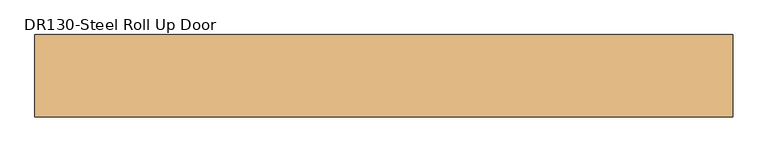
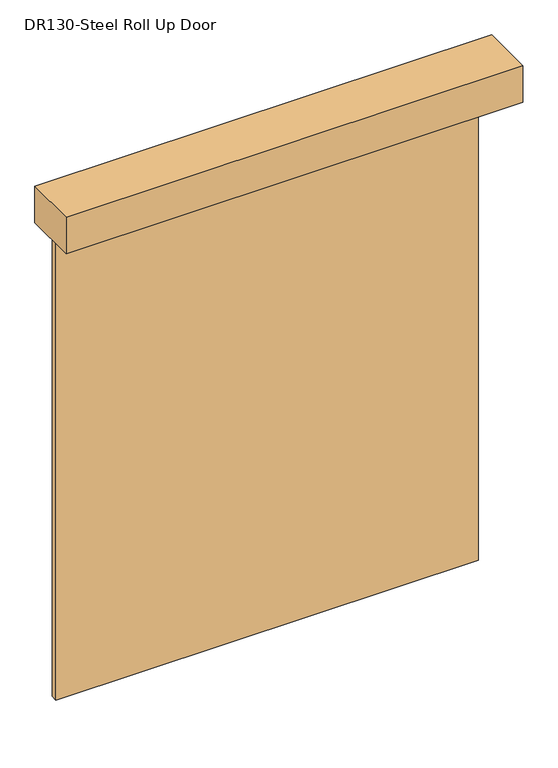
"""IFC4 building model written with IfcOpenShell, lengths in millimetres: door geometry, DR130-Steel Roll Up Door : DR131-Steel Roll Up Door-W4000xH4000mm."""

from ifc_helpers import new_model, si_unit, frame, origin, origin_with_axes, place, context, project, spatial, polyline, outline, extrude, source, transform, mapped, element, save


def dr130_steel_roll_up_door_e99b7ff9(model_context):
    return source(origin(), model_context, "Body", "SweptSolid", [
        extrude(outline(polyline([(2703.2, -858.8), (-2703.2, -858.8), (-2703.2, -220.0), (2703.2, -220.0), (2703.2, -858.8)])), frame((0.0, 0.0, 6000.0), z_axis=(0.0, 0.0, 1.0), x_axis=(1.0, 0.0, 0.0)), (0.0, 0.0, 1.0), 457.2),
        extrude(outline(polyline([(2500.0, -220.0), (2500.0, -300.0), (-2500.0, -300.0), (-2500.0, -220.0), (2500.0, -220.0)])), origin_with_axes(), (0.0, 0.0, 1.0), 6000.0),
    ])


if __name__ == "__main__":
    model = new_model("IFC4")
    model_context = context("Model", 3, world=origin())
    ifc_project = project(units=[si_unit("LENGTHUNIT", "METRE", prefix="MILLI")], contexts=[model_context])
    site = spatial("IfcSite", under=ifc_project)
    building = spatial("IfcBuilding", under=site)
    placement = place(None, origin())
    dr130_steel_roll_up_door_shape = dr130_steel_roll_up_door_e99b7ff9(model_context)
    element("IfcDoor", 1, ObjectType="DR130-Steel Roll Up Door : DR131-Steel Roll Up Door-W4000xH4000mm", at=placement, inside=building, context=model_context, shape_type="MappedRepresentation", body=[
        mapped(dr130_steel_roll_up_door_shape, transform((0.0, 0.0, 0.0), x_axis=(1.0, 0.0, 0.0), y_axis=(0.0, 1.0, 0.0), z_axis=(0.0, 0.0, 1.0))),
    ])
    save(model, "model.ifc")

# Revit data of these elements
# Type "DR130-Steel Roll Up Door : DR131-Steel Roll Up Door-W4000xH4000mm"
#   Type Mark = "362"
#   Construction Type Id = "MDOOR"
#   Assembly Code = "B2030400"
#   Analytic Construction = "<None>"
#   Thickness = 0.0800 m
#   Thermal Resistance (R) = 0.270117 (m²·K)/W
#   Rough Width [instance default] = 4.0000 m
#   Rough Height [instance default] = 4.0000 m
#   Offset [instance default] = 1.0000 m
#   Heat Transfer Coefficient (U) = 3.7021 W/(m²·K)
#   Height [instance default] = 4.0000 m
#   Width [instance default] = 4.0000 m
#   Function = 1
#   Define Thermal Properties by = 1
#   Canopy [instance default] = yes
#   Roller Material = A04AQ112-00002_Steel Roll Up Door
#   Roller Box Material = A04AQ112-00002_Steel Roll Up Door
#   Visual Light Transmittance = 0
#   Solar Heat Gain Coefficient = 0
#   Wall Closure = (empty or 0)
# Element 1 (IfcDoor, "DR130-Steel Roll Up Door : DR131-Steel Roll Up Door-W4000xH4000mm")
#   Rough Width = 5.0000 m
#   Rough Height = 6.0000 m
#   Offset = 0.2600 m
#   Height = 6.0000 m
#   Width = 5.0000 m
#   Canopy = no
#   Materials on its faces: "A04AQ112-00002_Steel Roll Up Door"
# Materials
#   "A04AQ112-00002_Steel Roll Up Door": class "금속", colour RGB 247 247 247, transparency 0, Description = "Steel Door", Cost = 0
